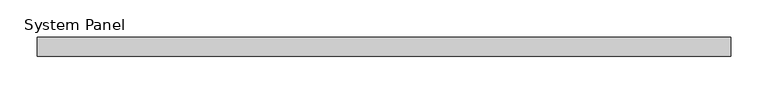
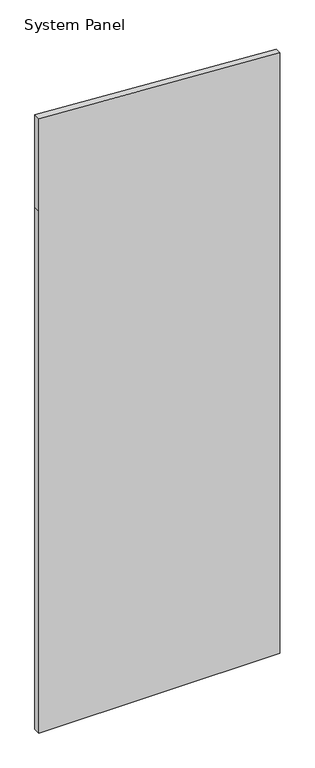
"""IFC4 building model written with IfcOpenShell, lengths in millimetres: plate geometry, System Panel : TEMPERED INSULATED GLAZING (CARDINAL GLASS LoĒ²-240."""

from ifc_helpers import new_model, si_unit, frame, origin, place, context, project, spatial, polyline, outline, extrude, source, transform, mapped, element, save


def system_panel_4f0ef3e2(model_context):
    return source(origin(), model_context, "Body", "SweptSolid", [
        extrude(outline(polyline([(0.0, -464.740625), (0.0, 464.740625), (2127.25, 464.740625), (2446.7344717, 464.740625), (2504.8270498, -464.740625), (2127.25, -464.740625), (0.0, -464.740625)])), frame((0.0, 6.35, 0.0), z_axis=(0.0, 1.0, 0.0), x_axis=(0.0, 0.0, 1.0)), (0.0, 0.0, 1.0), 25.4),
    ])


if __name__ == "__main__":
    model = new_model("IFC4")
    model_context = context("Model", 3, world=origin())
    ifc_project = project(units=[si_unit("LENGTHUNIT", "METRE", prefix="MILLI")], contexts=[model_context])
    site = spatial("IfcSite", under=ifc_project)
    building = spatial("IfcBuilding", under=site)
    placement = place(None, origin())
    system_panel_shape = system_panel_4f0ef3e2(model_context)
    element("IfcPlate", 1, ObjectType="System Panel : TEMPERED INSULATED GLAZING (CARDINAL GLASS LoĒ²-240", at=placement, inside=building, context=model_context, shape_type="MappedRepresentation", body=[
        mapped(system_panel_shape, transform((0.0, 0.0, 0.0), x_axis=(1.0, 0.0, 0.0), y_axis=(0.0, 1.0, 0.0), z_axis=(0.0, 0.0, 1.0))),
    ])
    save(model, "model.ifc")

# Revit data of these elements
# Type "System Panel : TEMPERED INSULATED GLAZING (CARDINAL GLASS LoĒ²-240"
#   Construction Type Id = "opn-s72"
#   Analytic Construction = "Double glazing - 1/4 in thick - low-E/clear (e = 0.1) glass"
#   Visual Light Transmittance = 0.72
#   Solar Heat Gain Coefficient = 0.6
#   Heat Transfer Coefficient (U) = 1.9873 W/(m²·K)
#   Transparency_Hack = 70
# Element 1 (IfcPlate, "System Panel : TEMPERED INSULATED GLAZING (CARDINAL GLASS LoĒ²-240")
#   Materials on its faces: "TEMPERED INSULATED GLAZING (CARDINAL GLASS LoĒ²-240\nOR EQUIVALENT)"
# Materials
#   "TEMPERED INSULATED GLAZING (CARDINAL GLASS LoĒ²-240\nOR EQUIVALENT)": class "Glass", colour RGB 196 205 210, transparency 0.85, Description = "Soda Lime Glass", Cost = 0
